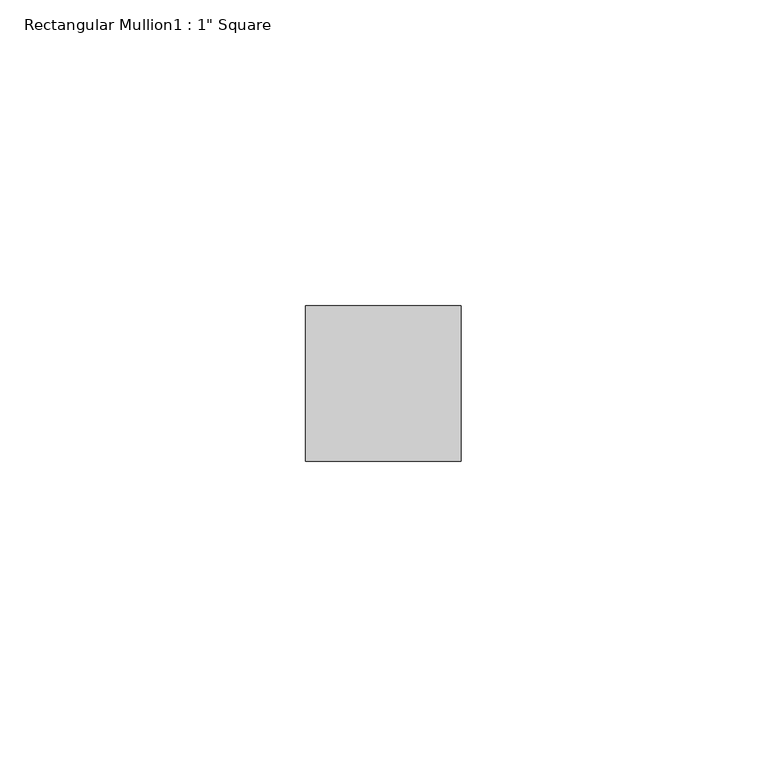
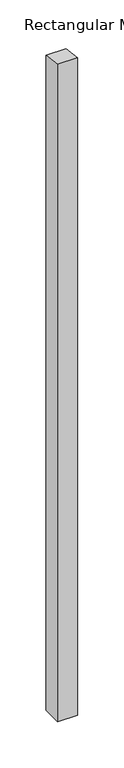
"""IFC4 building model written with IfcOpenShell, lengths in millimetres: member geometry."""

import ifcopenshell
import ifcopenshell.guid

model = None  # the IFC model being written
_history = None  # IfcOwnerHistory: only IFC2X3 demands one
_inside = {}  # id of a spatial element -> (the spatial element, [elements in it])
_under = {}  # id of a project, library or spatial element -> (it, [spatial elements below it])
_declared = {}  # id of a project -> (the project, [libraries it declares])
_typed = {}  # id of a type object -> (the type object, [elements of that type])
_made_of = {}  # id of a material, layer set ... -> (it, [elements and type objects made of it])


def new_model(schema):
    """Start an empty IFC model of exactly this schema.

    Asked for "IFC4X3", IfcOpenShell would pick the latest addendum, in which some entities
    have other attributes; the version numbers below select the first issue.
    IFC2X3 requires an IfcOwnerHistory on every rooted entity: one is made here for all.
    """
    global model, _history
    if schema == "IFC4X3":
        model = ifcopenshell.file(schema_version=(4, 3, 0, 0))
    else:
        model = ifcopenshell.file(schema=schema)
    _inside.clear()
    _under.clear()
    _declared.clear()
    _typed.clear()
    _made_of.clear()
    _history = None
    if model.schema == "IFC2X3":
        org = make("IfcOrganization", Name="unknown")
        user = make(
            "IfcPersonAndOrganization",
            ThePerson=make("IfcPerson", FamilyName="unknown"),
            TheOrganization=org,
        )
        app = make(
            "IfcApplication",
            ApplicationDeveloper=org,
            Version="unknown",
            ApplicationFullName="unknown",
            ApplicationIdentifier="unknown",
        )
        _history = make(
            "IfcOwnerHistory",
            OwningUser=user,
            OwningApplication=app,
            ChangeAction="ADDED",
            CreationDate=0,
        )
    return model


def make(cls, **values):
    """One entity of the class cls with the attributes given. An attribute that is None is left unset."""
    return model.create_entity(
        cls, **{name: value for name, value in values.items() if value is not None}
    )


def rooted(cls, **values):
    """An entity with a GlobalId (a new one), such as an element, a storey or a relation."""
    return make(cls, GlobalId=ifcopenshell.guid.new(), OwnerHistory=_history, **values)


def si_unit(unit_type, name, prefix=None):
    """IfcSIUnit, for example si_unit("LENGTHUNIT", "METRE", prefix="MILLI")."""
    return make("IfcSIUnit", UnitType=unit_type, Prefix=prefix, Name=name)


def assignment(units):
    """IfcUnitAssignment: the units of a project."""
    return None if units is None else make("IfcUnitAssignment", Units=units)


def point(xyz):
    """IfcCartesianPoint."""
    return None if xyz is None else make("IfcCartesianPoint", Coordinates=xyz)


def direction(xyz):
    """IfcDirection."""
    return None if xyz is None else make("IfcDirection", DirectionRatios=xyz)


def frame(location, z_axis=None, x_axis=None):
    """IfcAxis2Placement3D, a coordinate frame: its origin and axes. An axis left out is left unset."""
    return make(
        "IfcAxis2Placement3D",
        Location=point(location),
        Axis=direction(z_axis),
        RefDirection=direction(x_axis),
    )


def origin():
    """The frame at (0, 0, 0) with its axes left unset."""
    return frame((0.0, 0.0, 0.0))


def place(relative_to, where):
    """IfcLocalPlacement: puts the frame where relative to a parent placement (None: the world)."""
    return make(
        "IfcLocalPlacement", PlacementRelTo=relative_to, RelativePlacement=where
    )


def context(
    kind, dimensions, precision=None, world=None, true_north=None, identifier=None
):
    """IfcGeometricRepresentationContext, for example the 3D "Model" context."""
    return make(
        "IfcGeometricRepresentationContext",
        ContextIdentifier=identifier,
        ContextType=kind,
        CoordinateSpaceDimension=dimensions,
        Precision=precision,
        WorldCoordinateSystem=world,
        TrueNorth=true_north,
    )


def project(units=None, contexts=None):
    """IfcProject with its units and contexts."""
    return rooted(
        "IfcProject",
        Name="project",
        RepresentationContexts=contexts,
        UnitsInContext=assignment(units),
    )


def spatial(cls, under=None, at=None, **own):
    """A site, building, storey or space (cls), placed at a placement, below another one or the project."""
    s = rooted(cls, ObjectPlacement=at, **own)
    if under is not None:
        _under.setdefault(under.id(), (under, []))[1].append(s)
    return s


def polyline(points):
    """IfcPolyline through the points."""
    return make("IfcPolyline", Points=[point(p) for p in points])


def outline(outer, holes=None, kind="AREA"):
    """IfcArbitraryClosedProfileDef: a profile drawn as a closed curve; with holes, ...WithVoids."""
    if holes is None:
        return make("IfcArbitraryClosedProfileDef", ProfileType=kind, OuterCurve=outer)
    return make(
        "IfcArbitraryProfileDefWithVoids",
        ProfileType=kind,
        OuterCurve=outer,
        InnerCurves=holes,
    )


def extrude(swept, where, along, depth):
    """IfcExtrudedAreaSolid: the profile swept, set in the frame where, extruded along a direction by depth."""
    return make(
        "IfcExtrudedAreaSolid",
        SweptArea=swept,
        Position=where,
        ExtrudedDirection=direction(along),
        Depth=depth,
    )


def shape(context_of_items, identifier, shape_type, items):
    """IfcShapeRepresentation: the items that make up one representation, for example the "Body"."""
    return make(
        "IfcShapeRepresentation",
        ContextOfItems=context_of_items,
        RepresentationIdentifier=identifier,
        RepresentationType=shape_type,
        Items=items,
    )


def source(mapping_origin, context_of_items, identifier, shape_type, items):
    """IfcRepresentationMap: a shape defined once, which mapped items show again and again."""
    return make(
        "IfcRepresentationMap",
        MappingOrigin=mapping_origin,
        MappedRepresentation=shape(context_of_items, identifier, shape_type, items),
    )


def transform(
    local_origin,
    x_axis=None,
    y_axis=None,
    z_axis=None,
    scale=None,
    scale2=None,
    scale3=None,
    uniform=True,
):
    """IfcCartesianTransformationOperator3D, or its non-uniform kind. x_axis, y_axis, z_axis: its Axis1, 2, 3."""
    if uniform:
        return make(
            "IfcCartesianTransformationOperator3D",
            Axis1=direction(x_axis),
            Axis2=direction(y_axis),
            LocalOrigin=point(local_origin),
            Scale=scale,
            Axis3=direction(z_axis),
        )
    return make(
        "IfcCartesianTransformationOperator3DnonUniform",
        Axis1=direction(x_axis),
        Axis2=direction(y_axis),
        LocalOrigin=point(local_origin),
        Scale=scale,
        Axis3=direction(z_axis),
        Scale2=scale2,
        Scale3=scale3,
    )


def mapped(mapping_source, mapping_target):
    """IfcMappedItem: shows the shape of a source again, moved by a transform."""
    return make(
        "IfcMappedItem", MappingSource=mapping_source, MappingTarget=mapping_target
    )


def made_of(thing, what):
    """Note that an element or type object is made of a material, layer set ...; save() writes the relation."""
    if what is not None:
        _made_of.setdefault(what.id(), (what, []))[1].append(thing)
    return thing


def element(
    cls,
    number,
    at=None,
    inside=None,
    cuts=None,
    type_object=None,
    material=None,
    context=None,
    identifier="Body",
    shape_type=None,
    held_by="IfcProductDefinitionShape",
    body=None,
    shapes=None,
    **own,
):
    """One element of the class cls, such as IfcWall. Its Tag is "e" and its number.

    at: its placement. inside: the storey or other place that contains it. cuts: it is an
    opening in that element (IfcRelVoidsElement). A single representation is given by context,
    identifier, shape_type and body (its items); several are given by shapes. held_by: the class
    of the entity that holds the representations. save() writes the other relations.
    """
    e = rooted(cls, Tag="e%d" % number, ObjectPlacement=at, **own)
    if body is not None:
        shapes = [shape(context, identifier, shape_type, body)]
    if shapes is not None:
        e.Representation = make(held_by, Representations=shapes)
    if inside is not None:
        _inside.setdefault(inside.id(), (inside, []))[1].append(e)
    if cuts is not None:
        rooted(
            "IfcRelVoidsElement", RelatingBuildingElement=cuts, RelatedOpeningElement=e
        )
    if type_object is not None:
        _typed.setdefault(type_object.id(), (type_object, []))[1].append(e)
    return made_of(e, material)


def aggregate(whole, parts):
    """IfcRelAggregates: a whole, such as a stair, and the parts it consists of."""
    return rooted("IfcRelAggregates", RelatingObject=whole, RelatedObjects=parts)


def save(model, path):
    """Write the relations noted so far, then the file.

    IfcRelAggregates (storeys below a building ...), IfcRelContainedInSpatialStructure (elements
    in a storey), IfcRelDefinesByType, IfcRelAssociatesMaterial and IfcRelDeclares: one each for
    every whole, place, type object, material and project.
    """
    for whole, parts in _under.values():
        aggregate(whole, parts)
    for where, things in _inside.values():
        rooted(
            "IfcRelContainedInSpatialStructure",
            RelatedElements=things,
            RelatingStructure=where,
        )
    for kind, things in _typed.values():
        rooted("IfcRelDefinesByType", RelatedObjects=things, RelatingType=kind)
    for what, things in _made_of.values():
        rooted("IfcRelAssociatesMaterial", RelatedObjects=things, RelatingMaterial=what)
    for by, libraries in _declared.values():
        rooted("IfcRelDeclares", RelatingContext=by, RelatedDefinitions=libraries)
    model.write(path)


def member_a9d6c361(model_context):
    return source(origin(), model_context, "Body", "SweptSolid", [
        extrude(outline(polyline([(-44.45, 5.7962627), (-19.05, 2.4841126), (-19.05, -866.1779877), (-44.45, -866.1779877), (-44.45, 5.7962627)])), frame((-25.4, 0.0, 0.0), z_axis=(1.0, 0.0, 0.0), x_axis=(0.0, 1.0, 0.0)), (0.0, 0.0, 1.0), 25.4),
    ])


if __name__ == "__main__":
    model = new_model("IFC4")
    model_context = context("Model", 3, world=origin())
    ifc_project = project(units=[si_unit("LENGTHUNIT", "METRE", prefix="MILLI")], contexts=[model_context])
    site = spatial("IfcSite", under=ifc_project)
    building = spatial("IfcBuilding", under=site)
    placement = place(None, origin())
    member_shape = member_a9d6c361(model_context)
    element("IfcMember", 1, ObjectType="Rectangular Mullion1 : 1\" Square", at=placement, inside=building, context=model_context, shape_type="MappedRepresentation", body=[
        mapped(member_shape, transform((0.0, 0.0, 0.0), x_axis=(1.0, 0.0, 0.0), y_axis=(0.0, 1.0, 0.0), z_axis=(0.0, 0.0, 1.0))),
    ])
    save(model, "model.ifc")

# Revit data of these elements
# Type "Rectangular Mullion1 : 1\" Square"
#   built-in parameter 1007351 = 0.104167 (stored number, unit not read)
#   built-in parameter 1007304 = 0.0833333 (stored number, unit not read)
#   built-in parameter 1007301 = 0.0416667 (stored number, unit not read)
#   built-in parameter 1007300 = 0.0416667 (stored number, unit not read)
